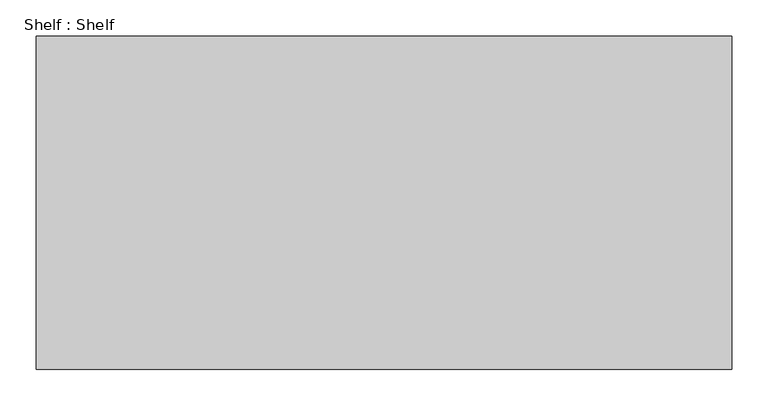
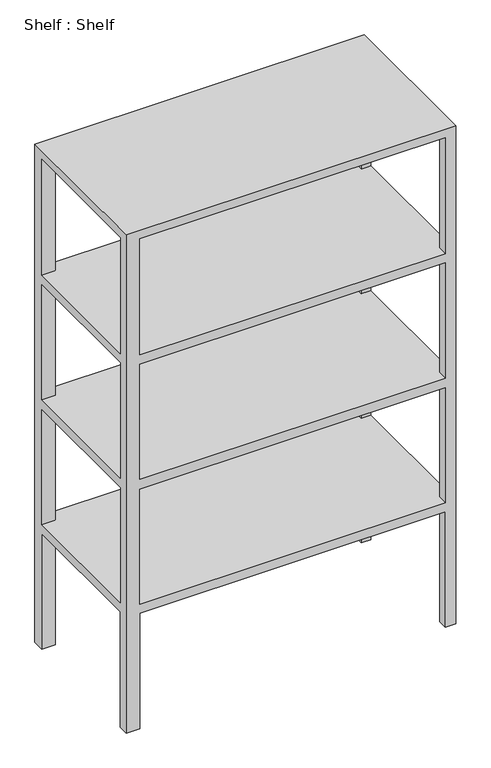
"""IFC4 building model written with IfcOpenShell, lengths in millimetres: furniture geometry, Shelf : Shelf."""

import ifcopenshell
import ifcopenshell.guid

model = None  # the IFC model being written
_history = None  # IfcOwnerHistory: only IFC2X3 demands one
_inside = {}  # id of a spatial element -> (the spatial element, [elements in it])
_under = {}  # id of a project, library or spatial element -> (it, [spatial elements below it])
_declared = {}  # id of a project -> (the project, [libraries it declares])
_typed = {}  # id of a type object -> (the type object, [elements of that type])
_made_of = {}  # id of a material, layer set ... -> (it, [elements and type objects made of it])


def new_model(schema):
    """Start an empty IFC model of exactly this schema.

    Asked for "IFC4X3", IfcOpenShell would pick the latest addendum, in which some entities
    have other attributes; the version numbers below select the first issue.
    IFC2X3 requires an IfcOwnerHistory on every rooted entity: one is made here for all.
    """
    global model, _history
    if schema == "IFC4X3":
        model = ifcopenshell.file(schema_version=(4, 3, 0, 0))
    else:
        model = ifcopenshell.file(schema=schema)
    _inside.clear()
    _under.clear()
    _declared.clear()
    _typed.clear()
    _made_of.clear()
    _history = None
    if model.schema == "IFC2X3":
        org = make("IfcOrganization", Name="unknown")
        user = make(
            "IfcPersonAndOrganization",
            ThePerson=make("IfcPerson", FamilyName="unknown"),
            TheOrganization=org,
        )
        app = make(
            "IfcApplication",
            ApplicationDeveloper=org,
            Version="unknown",
            ApplicationFullName="unknown",
            ApplicationIdentifier="unknown",
        )
        _history = make(
            "IfcOwnerHistory",
            OwningUser=user,
            OwningApplication=app,
            ChangeAction="ADDED",
            CreationDate=0,
        )
    return model


def make(cls, **values):
    """One entity of the class cls with the attributes given. An attribute that is None is left unset."""
    return model.create_entity(
        cls, **{name: value for name, value in values.items() if value is not None}
    )


def rooted(cls, **values):
    """An entity with a GlobalId (a new one), such as an element, a storey or a relation."""
    return make(cls, GlobalId=ifcopenshell.guid.new(), OwnerHistory=_history, **values)


def si_unit(unit_type, name, prefix=None):
    """IfcSIUnit, for example si_unit("LENGTHUNIT", "METRE", prefix="MILLI")."""
    return make("IfcSIUnit", UnitType=unit_type, Prefix=prefix, Name=name)


def assignment(units):
    """IfcUnitAssignment: the units of a project."""
    return None if units is None else make("IfcUnitAssignment", Units=units)


def point(xyz):
    """IfcCartesianPoint."""
    return None if xyz is None else make("IfcCartesianPoint", Coordinates=xyz)


def direction(xyz):
    """IfcDirection."""
    return None if xyz is None else make("IfcDirection", DirectionRatios=xyz)


def frame(location, z_axis=None, x_axis=None):
    """IfcAxis2Placement3D, a coordinate frame: its origin and axes. An axis left out is left unset."""
    return make(
        "IfcAxis2Placement3D",
        Location=point(location),
        Axis=direction(z_axis),
        RefDirection=direction(x_axis),
    )


def origin():
    """The frame at (0, 0, 0) with its axes left unset."""
    return frame((0.0, 0.0, 0.0))


def place(relative_to, where):
    """IfcLocalPlacement: puts the frame where relative to a parent placement (None: the world)."""
    return make(
        "IfcLocalPlacement", PlacementRelTo=relative_to, RelativePlacement=where
    )


def context(
    kind, dimensions, precision=None, world=None, true_north=None, identifier=None
):
    """IfcGeometricRepresentationContext, for example the 3D "Model" context."""
    return make(
        "IfcGeometricRepresentationContext",
        ContextIdentifier=identifier,
        ContextType=kind,
        CoordinateSpaceDimension=dimensions,
        Precision=precision,
        WorldCoordinateSystem=world,
        TrueNorth=true_north,
    )


def project(units=None, contexts=None):
    """IfcProject with its units and contexts."""
    return rooted(
        "IfcProject",
        Name="project",
        RepresentationContexts=contexts,
        UnitsInContext=assignment(units),
    )


def spatial(cls, under=None, at=None, **own):
    """A site, building, storey or space (cls), placed at a placement, below another one or the project."""
    s = rooted(cls, ObjectPlacement=at, **own)
    if under is not None:
        _under.setdefault(under.id(), (under, []))[1].append(s)
    return s


def faces_of(points, faces, orient=None, outer=None):
    """IfcFace entities. A face is a list of loops; a loop is a list of indices into points, from 0.

    orient and outer hold one flag for each loop. By default every Orientation is true, the
    first loop of a face is its IfcFaceOuterBound and the others are IfcFaceBound.
    """
    made = []
    for i, loops in enumerate(faces):
        bounds = []
        for j, loop in enumerate(loops):
            is_outer = j == 0 if outer is None else outer[i][j]
            bounds.append(
                make(
                    "IfcFaceOuterBound" if is_outer else "IfcFaceBound",
                    Bound=make("IfcPolyLoop", Polygon=[points[k] for k in loop]),
                    Orientation=True if orient is None else orient[i][j],
                )
            )
        made.append(make("IfcFace", Bounds=bounds))
    return made


def faceted_brep(points, faces, orient=None, outer=None, voids=None):
    """IfcFacetedBrep: a solid bounded by flat faces; with voids (closed shells), ...WithVoids."""
    shared = [point(p) for p in points]
    hull = make("IfcClosedShell", CfsFaces=faces_of(shared, faces, orient, outer))
    if voids is None:
        return make("IfcFacetedBrep", Outer=hull)
    return make(
        "IfcFacetedBrepWithVoids",
        Outer=hull,
        Voids=[
            make(cls, CfsFaces=faces_of(shared, fs, o, b)) for cls, fs, o, b in voids
        ],
    )


def shape(context_of_items, identifier, shape_type, items):
    """IfcShapeRepresentation: the items that make up one representation, for example the "Body"."""
    return make(
        "IfcShapeRepresentation",
        ContextOfItems=context_of_items,
        RepresentationIdentifier=identifier,
        RepresentationType=shape_type,
        Items=items,
    )


def source(mapping_origin, context_of_items, identifier, shape_type, items):
    """IfcRepresentationMap: a shape defined once, which mapped items show again and again."""
    return make(
        "IfcRepresentationMap",
        MappingOrigin=mapping_origin,
        MappedRepresentation=shape(context_of_items, identifier, shape_type, items),
    )


def transform(
    local_origin,
    x_axis=None,
    y_axis=None,
    z_axis=None,
    scale=None,
    scale2=None,
    scale3=None,
    uniform=True,
):
    """IfcCartesianTransformationOperator3D, or its non-uniform kind. x_axis, y_axis, z_axis: its Axis1, 2, 3."""
    if uniform:
        return make(
            "IfcCartesianTransformationOperator3D",
            Axis1=direction(x_axis),
            Axis2=direction(y_axis),
            LocalOrigin=point(local_origin),
            Scale=scale,
            Axis3=direction(z_axis),
        )
    return make(
        "IfcCartesianTransformationOperator3DnonUniform",
        Axis1=direction(x_axis),
        Axis2=direction(y_axis),
        LocalOrigin=point(local_origin),
        Scale=scale,
        Axis3=direction(z_axis),
        Scale2=scale2,
        Scale3=scale3,
    )


def mapped(mapping_source, mapping_target):
    """IfcMappedItem: shows the shape of a source again, moved by a transform."""
    return make(
        "IfcMappedItem", MappingSource=mapping_source, MappingTarget=mapping_target
    )


def made_of(thing, what):
    """Note that an element or type object is made of a material, layer set ...; save() writes the relation."""
    if what is not None:
        _made_of.setdefault(what.id(), (what, []))[1].append(thing)
    return thing


def element(
    cls,
    number,
    at=None,
    inside=None,
    cuts=None,
    type_object=None,
    material=None,
    context=None,
    identifier="Body",
    shape_type=None,
    held_by="IfcProductDefinitionShape",
    body=None,
    shapes=None,
    **own,
):
    """One element of the class cls, such as IfcWall. Its Tag is "e" and its number.

    at: its placement. inside: the storey or other place that contains it. cuts: it is an
    opening in that element (IfcRelVoidsElement). A single representation is given by context,
    identifier, shape_type and body (its items); several are given by shapes. held_by: the class
    of the entity that holds the representations. save() writes the other relations.
    """
    e = rooted(cls, Tag="e%d" % number, ObjectPlacement=at, **own)
    if body is not None:
        shapes = [shape(context, identifier, shape_type, body)]
    if shapes is not None:
        e.Representation = make(held_by, Representations=shapes)
    if inside is not None:
        _inside.setdefault(inside.id(), (inside, []))[1].append(e)
    if cuts is not None:
        rooted(
            "IfcRelVoidsElement", RelatingBuildingElement=cuts, RelatedOpeningElement=e
        )
    if type_object is not None:
        _typed.setdefault(type_object.id(), (type_object, []))[1].append(e)
    return made_of(e, material)


def aggregate(whole, parts):
    """IfcRelAggregates: a whole, such as a stair, and the parts it consists of."""
    return rooted("IfcRelAggregates", RelatingObject=whole, RelatedObjects=parts)


def save(model, path):
    """Write the relations noted so far, then the file.

    IfcRelAggregates (storeys below a building ...), IfcRelContainedInSpatialStructure (elements
    in a storey), IfcRelDefinesByType, IfcRelAssociatesMaterial and IfcRelDeclares: one each for
    every whole, place, type object, material and project.
    """
    for whole, parts in _under.values():
        aggregate(whole, parts)
    for where, things in _inside.values():
        rooted(
            "IfcRelContainedInSpatialStructure",
            RelatedElements=things,
            RelatingStructure=where,
        )
    for kind, things in _typed.values():
        rooted("IfcRelDefinesByType", RelatedObjects=things, RelatingType=kind)
    for what, things in _made_of.values():
        rooted("IfcRelAssociatesMaterial", RelatedObjects=things, RelatingMaterial=what)
    for by, libraries in _declared.values():
        rooted("IfcRelDeclares", RelatingContext=by, RelatedDefinitions=libraries)
    model.write(path)


def shelf_shelf_d39eace1(model_context):
    return source(origin(), model_context, "Body", "Brep", [
        faceted_brep([(14056.7001442, 3277.8615366, 1524.0), (13103.4798744, 3277.8615366, 1524.0), (13103.4798744, 2820.6615366, 1524.0), (14056.7001442, 2820.6615366, 1524.0), (14056.7001442, 2849.585331, 0.0), (14056.7001442, 2820.6615366, 0.0), (14027.0281946, 2820.6615366, 0.0), (14027.0281946, 2849.585331, 0.0), (14056.7001442, 3277.8615366, 0.0), (14056.7001442, 3245.3048936, 0.0), (14028.3529362, 3245.3048936, 0.0), (14028.3529362, 3277.8615366, 0.0), (13142.3001442, 2820.6615366, 0.0), (13103.4798744, 2820.6615366, 0.0), (13103.4798744, 2849.585331, 0.0), (13142.3001442, 2849.585331, 0.0), (13103.4798744, 3244.0675604, 0.0), (13103.4798744, 3277.8615366, 0.0), (13142.3001442, 3277.8615366, 0.0), (13142.3001442, 3244.0675604, 0.0), (14028.3529362, 3277.8615366, 353.3332002), (13142.3001442, 3277.8615366, 353.3332002), (14028.3529362, 3277.8615366, 1497.6781444), (13142.3001442, 3277.8615366, 1497.6781444), (13142.3001442, 3277.8615366, 1143.0), (14028.3529362, 3277.8615366, 1143.0), (14028.3529362, 3277.8615366, 1114.8196695), (13142.3001442, 3277.8615366, 1114.8196695), (13142.3001442, 3277.8615366, 762.0), (14028.3529362, 3277.8615366, 762.0), (14028.3529362, 3277.8615366, 731.9611947), (13142.3001442, 3277.8615366, 731.9611947), (13142.3001442, 3277.8615366, 381.0), (14028.3529362, 3277.8615366, 381.0), (13103.4798744, 3244.0675604, 353.3332002), (13103.4798744, 2849.585331, 353.3332002), (13103.4798744, 3244.0675604, 1497.6781444), (13103.4798744, 2849.585331, 1497.6781444), (13103.4798744, 2849.585331, 1143.0), (13103.4798744, 3244.0675604, 1143.0), (13103.4798744, 3244.0675604, 1114.8196695), (13103.4798744, 2849.585331, 1114.8196695), (13103.4798744, 2849.585331, 762.0), (13103.4798744, 3244.0675604, 762.0), (13103.4798744, 3244.0675604, 731.9611947), (13103.4798744, 2849.585331, 731.9611947), (13103.4798744, 2849.585331, 381.0), (13103.4798744, 3244.0675604, 381.0), (13142.3001442, 2820.6615366, 353.3332002), (14027.0281946, 2820.6615366, 353.3332002), (13142.3001442, 2820.6615366, 1497.6781444), (14027.0281946, 2820.6615366, 1497.6781444), (14027.0281946, 2820.6615366, 1143.0), (13142.3001442, 2820.6615366, 1143.0), (13142.3001442, 2820.6615366, 1114.8196695), (14027.0281946, 2820.6615366, 1114.8196695), (14027.0281946, 2820.6615366, 762.0), (13142.3001442, 2820.6615366, 762.0), (13142.3001442, 2820.6615366, 731.9611947), (14027.0281946, 2820.6615366, 731.9611947), (14027.0281946, 2820.6615366, 381.0), (13142.3001442, 2820.6615366, 381.0), (14056.7001442, 2849.585331, 353.3332002), (14056.7001442, 3245.3048936, 353.3332002), (14056.7001442, 2849.585331, 1497.6781444), (14056.7001442, 3245.3048936, 1497.6781444), (14056.7001442, 3245.3048936, 1143.0), (14056.7001442, 2849.585331, 1143.0), (14056.7001442, 2849.585331, 1114.8196695), (14056.7001442, 3245.3048936, 1114.8196695), (14056.7001442, 3245.3048936, 762.0), (14056.7001442, 2849.585331, 762.0), (14056.7001442, 2849.585331, 731.9611947), (14056.7001442, 3245.3048936, 731.9611947), (14056.7001442, 3245.3048936, 381.0), (14056.7001442, 2849.585331, 381.0), (13142.3001442, 2849.585331, 1497.6781444), (13142.3001442, 3244.0675604, 1497.6781444), (14028.3529362, 3245.3048936, 1497.6781444), (14027.0281946, 2849.585331, 1497.6781444), (13142.3001442, 2849.585331, 1143.0), (14027.0281946, 2849.585331, 1143.0), (14028.3529362, 3245.3048936, 1143.0), (13142.3001442, 3244.0675604, 1143.0), (13142.3001442, 2849.585331, 1114.8196695), (13142.3001442, 3244.0675604, 1114.8196695), (14028.3529362, 3245.3048936, 1114.8196695), (14027.0281946, 2849.585331, 1114.8196695), (13142.3001442, 2849.585331, 762.0), (14027.0281946, 2849.585331, 762.0), (14028.3529362, 3245.3048936, 762.0), (13142.3001442, 3244.0675604, 762.0), (13142.3001442, 2849.585331, 731.9611947), (13142.3001442, 3244.0675604, 731.9611947), (14028.3529362, 3245.3048936, 731.9611947), (14027.0281946, 2849.585331, 731.9611947), (13142.3001442, 2849.585331, 381.0), (14027.0281946, 2849.585331, 381.0), (14028.3529362, 3245.3048936, 381.0), (13142.3001442, 3244.0675604, 381.0), (13142.3001442, 2849.585331, 353.3332002), (13142.3001442, 3244.0675604, 353.3332002), (14028.3529362, 3245.3048936, 353.3332002), (14027.0281946, 2849.585331, 353.3332002)], [[[0, 1, 2, 3]], [[4, 5, 6, 7]], [[8, 9, 10, 11]], [[12, 13, 14, 15]], [[16, 17, 18, 19]], [[1, 0, 8, 11, 20, 21, 18, 17], [22, 23, 24, 25], [26, 27, 28, 29], [30, 31, 32, 33]], [[2, 1, 17, 16, 34, 35, 14, 13], [36, 37, 38, 39], [40, 41, 42, 43], [44, 45, 46, 47]], [[3, 2, 13, 12, 48, 49, 6, 5], [50, 51, 52, 53], [54, 55, 56, 57], [58, 59, 60, 61]], [[0, 3, 5, 4, 62, 63, 9, 8], [64, 65, 66, 67], [68, 69, 70, 71], [72, 73, 74, 75]], [[76, 37, 36, 77, 23, 22, 78, 65, 64, 79, 51, 50]], [[80, 53, 52, 81, 67, 66, 82, 25, 24, 83, 39, 38]], [[76, 50, 53, 80]], [[51, 79, 81, 52]], [[79, 64, 67, 81]], [[65, 78, 82, 66]], [[78, 22, 25, 82]], [[23, 77, 83, 24]], [[77, 36, 39, 83]], [[37, 76, 80, 38]], [[84, 41, 40, 85, 27, 26, 86, 69, 68, 87, 55, 54]], [[88, 57, 56, 89, 71, 70, 90, 29, 28, 91, 43, 42]], [[84, 54, 57, 88]], [[55, 87, 89, 56]], [[87, 68, 71, 89]], [[69, 86, 90, 70]], [[86, 26, 29, 90]], [[27, 85, 91, 28]], [[85, 40, 43, 91]], [[41, 84, 88, 42]], [[92, 45, 44, 93, 31, 30, 94, 73, 72, 95, 59, 58]], [[96, 61, 60, 97, 75, 74, 98, 33, 32, 99, 47, 46]], [[92, 58, 61, 96]], [[59, 95, 97, 60]], [[95, 72, 75, 97]], [[73, 94, 98, 74]], [[94, 30, 33, 98]], [[31, 93, 99, 32]], [[93, 44, 47, 99]], [[45, 92, 96, 46]], [[100, 35, 34, 101, 21, 20, 102, 63, 62, 103, 49, 48]], [[100, 48, 12, 15]], [[49, 103, 7, 6]], [[103, 62, 4, 7]], [[63, 102, 10, 9]], [[102, 20, 11, 10]], [[21, 101, 19, 18]], [[101, 34, 16, 19]], [[35, 100, 15, 14]]]),
    ])


if __name__ == "__main__":
    model = new_model("IFC4")
    model_context = context("Model", 3, world=origin())
    ifc_project = project(units=[si_unit("LENGTHUNIT", "METRE", prefix="MILLI")], contexts=[model_context])
    site = spatial("IfcSite", under=ifc_project)
    building = spatial("IfcBuilding", under=site)
    placement = place(None, origin())
    shelf_shelf_shape = shelf_shelf_d39eace1(model_context)
    element("IfcFurniture", 1, ObjectType="Shelf : Shelf", at=placement, inside=building, context=model_context, shape_type="MappedRepresentation", body=[
        mapped(shelf_shelf_shape, transform((0.0, 0.0, 0.0), x_axis=(1.0, 0.0, 0.0), y_axis=(0.0, 1.0, 0.0), z_axis=(0.0, 0.0, 1.0))),
    ])
    save(model, "model.ifc")
